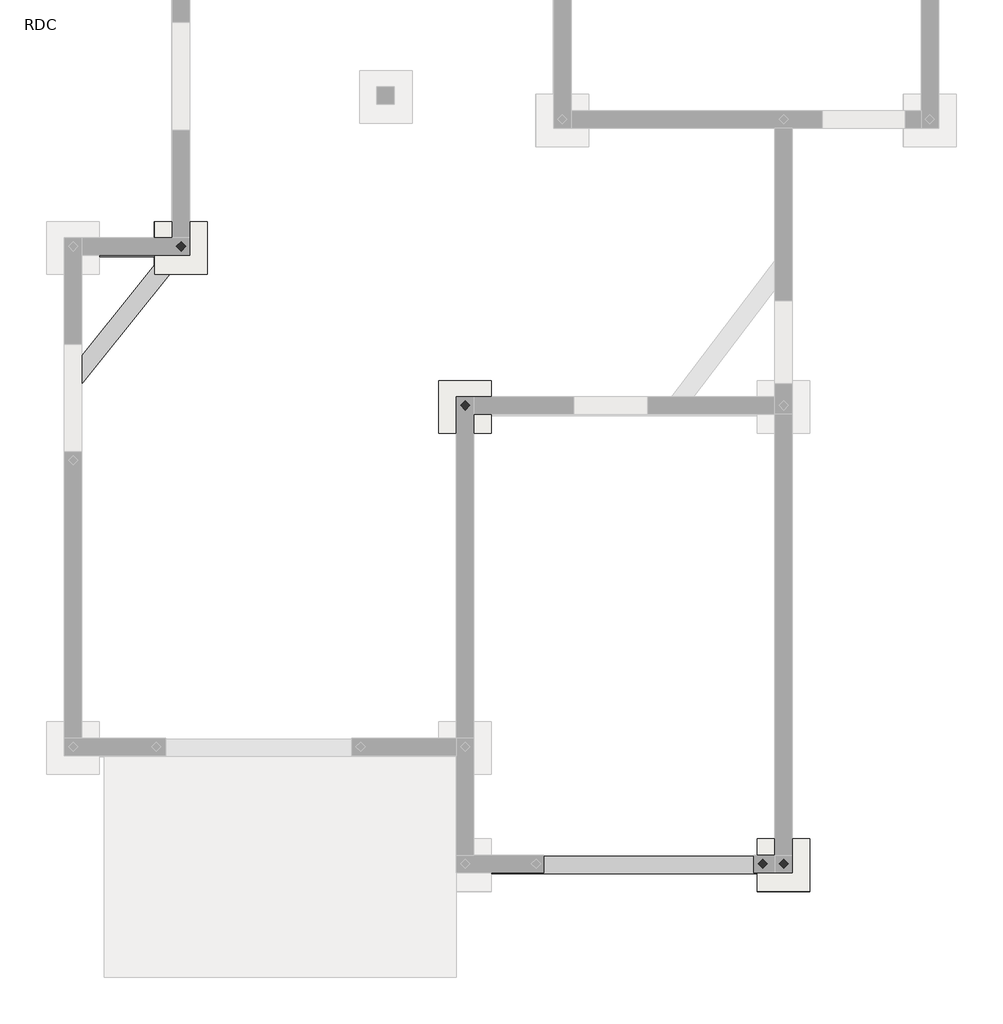
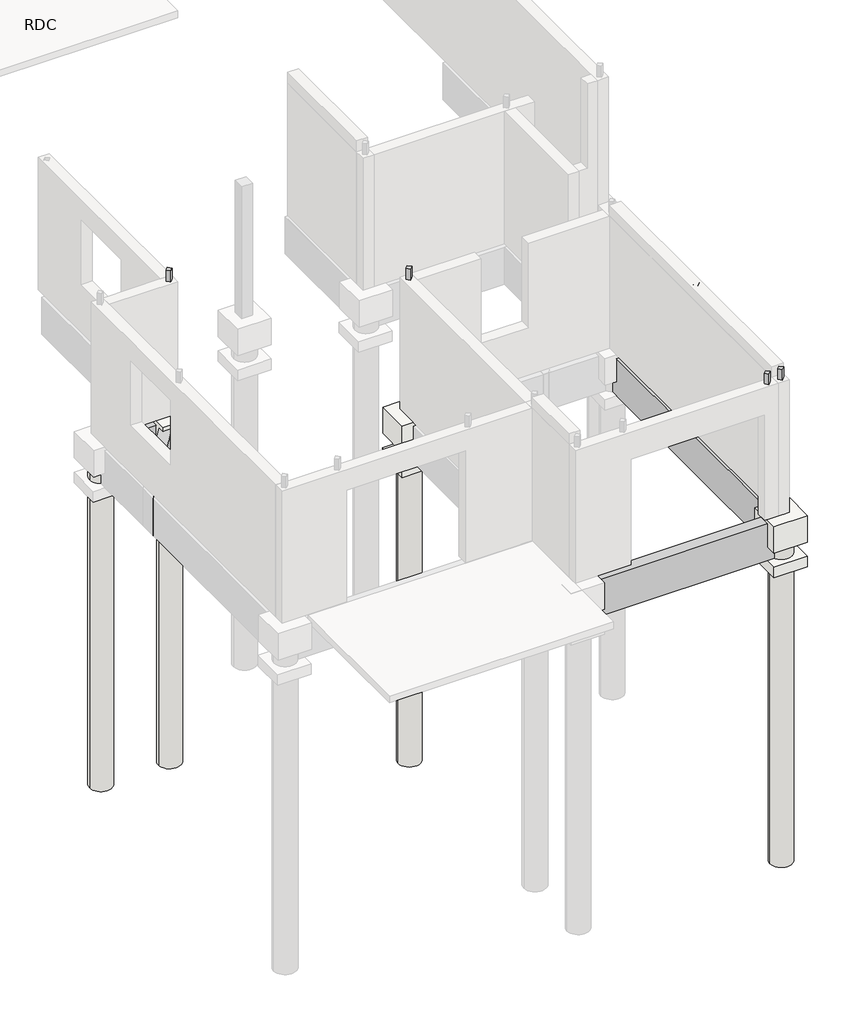
# One storey, part 3 of 5: 10 slabs, 5 columns, 4 beams.
"""IFC4 building model written with IfcOpenShell, lengths in millimetres."""

from ifc_helpers import new_model, si_unit, frame, origin, place, context, project, spatial, polyline, circle_curve, outline, extrude, faceted_brep, element, save
from ifc_brep_helpers import plane_surface, cylinder_surface, revolved_surface, advanced_brep

model = new_model("IFC4")

# Units and contexts
model_context = context("Model", 3, world=origin())
ifc_project = project(units=[si_unit("LENGTHUNIT", "METRE", prefix="MILLI")], contexts=[model_context])

# Site, building, storey
site = spatial("IfcSite", under=ifc_project)
building = spatial("IfcBuilding", under=site)
storey = spatial("IfcBuildingStorey", under=building, Name="RDC", Elevation=0.0)

# Beams
placement = place(None, origin())
element("IfcBeam", 1, ObjectType="Longrine BA : 20x70ht", at=placement, inside=storey, context=model_context, shape_type="AdvancedBrep", body=[
    advanced_brep(
    [(-6246.4904447, -2429.4243416, -767.0), (-6246.4904447, -2429.4243416, -67.0), (-5212.6214092, -1137.6788036, -67.0), (-5212.6214092, -1137.6788036, -500.0), (-5104.1092044, -1002.1005519, -500.0), (-5104.1092044, -1002.1005519, -767.0), (-4957.6914228, -1139.2289701, -767.0), (-6246.4904447, -2749.4913232, -767.0), (-6246.4904447, -2749.4913232, -67.0), (-4957.6914228, -1139.2289701, -500.0), (-5041.8454341, -1244.3733983, -500.0), (-5041.8454341, -1244.3733983, -67.0), (-5212.6214092, -1244.3733983, -67.0), (-5212.6214092, -1244.3733983, -500.0)],
    [
        (0, 1),
        (1, 2),
        (2, 3),
        (3, 4),
        (4, 5),
        (5, 0),
        (5, 6, circle_curve(frame((-4912.6214092, -944.3733983, -767.0), z_axis=(0.0, 0.0, 1.0), x_axis=(1.0, 0.0, 0.0)), 200.0)),
        (6, 7),
        (7, 0),
        (8, 7),
        (6, 9),
        (9, 10),
        (10, 11),
        (11, 8),
        (1, 8),
        (11, 12),
        (12, 2),
        (4, 9, circle_curve(frame((-4912.6214092, -944.3733983, -500.0), z_axis=(0.0, 0.0, 1.0), x_axis=(1.0, 0.0, 0.0)), 200.0)),
        (3, 13),
        (13, 10),
        (12, 13),
    ],
    [
        plane_surface(frame((-6038.5546058, -2169.6233583, -67.0), z_axis=(-0.780729452475571, 0.6248692039436695, 0.0), x_axis=(0.6248692039436695, 0.780729452475571, 0.0))),
        plane_surface(frame((-6038.5546058, -2169.6233583, -767.0), z_axis=(0.0, 0.0, -1.0000000000000002), x_axis=(0.6248692039436695, 0.780729452475571, 0.0))),
        plane_surface(frame((-5882.4087153, -2294.5971991, -767.0), z_axis=(0.780729452475571, -0.6248692039436695, 0.0), x_axis=(0.6248692039436695, 0.780729452475571, 0.0))),
        plane_surface(frame((-5882.4087153, -2294.5971991, -67.0), z_axis=(0.0, 0.0, 1.0000000000000002), x_axis=(0.6248692039436695, 0.780729452475571, 0.0))),
        revolved_surface(polyline([(-4712.6214092, -944.3733983, -500.0), (-4712.6214092, -944.3733983, -767.0)]), (-4912.6214092, -944.3733983, -6600.0), (0.0, 0.0, 1.0)),
        plane_surface(frame((-6246.4904447, -2766.3120846, -67.0), z_axis=(-1.0, 0.0, 0.0), x_axis=(0.0, 1.0, 0.0))),
        plane_surface(frame((-5212.6214092, -644.3733983, -500.0), z_axis=(0.0, 0.0, 1.0), x_axis=(1.0, 0.0, 0.0))),
        plane_surface(frame((-5212.6214092, -644.3733983, 0.0), z_axis=(1.0, 0.0, 0.0), x_axis=(0.0, 0.0, -1.0))),
        plane_surface(frame((-5212.6214092, -1244.3733983, 0.0), z_axis=(0.0, 1.0, 0.0), x_axis=(0.0, 0.0, -1.0))),
    ],
    [
        (0, [[1, 2, 3, 4, 5, 6]]),
        (1, [[7, 8, 9, -6]]),
        (2, [[10, -8, 11, 12, 13, 14]]),
        (3, [[15, -14, 16, 17, -2]]),
        (4, [[-7, -5, 18, -11]]),
        (5, [[-1, -9, -10, -15]]),
        (6, [[19, 20, -12, -18, -4]]),
        (7, [[-19, -3, -17, 21]]),
        (8, [[-20, -21, -16, -13]]),
    ],
),
])
element("IfcBeam", 2, ObjectType="Longrine BA : 20x70ht", at=placement, inside=storey, context=model_context, shape_type="AdvancedBrep", body=[
    advanced_brep(
    [(1796.8177589, -8101.9775185, -767.0), (1796.8177589, -8101.9775185, -500.0), (1670.0228479, -8101.9775185, -500.0), (1670.0228479, -8101.9775185, -67.0), (-1366.4904447, -8101.9775185, -67.0), (-1366.4904447, -8101.9775185, -500.0), (-1493.285364, -8101.9775185, -500.0), (-1493.285364, -8101.9775185, -767.0), (-1466.4904447, -8001.9775185, -767.0), (-1493.285364, -7901.9775185, -767.0), (1796.8177754, -7901.9775185, -767.0), (1770.0228479, -8001.9775328, -767.0), (1796.8177754, -7901.9775185, -500.0), (-1493.285364, -7901.9775185, -500.0), (-1366.4904447, -7901.9775185, -500.0), (-1366.4904447, -7901.9775185, -67.0), (1670.0228479, -7901.9775185, -67.0), (1670.0228479, -7901.9775185, -500.0), (-1466.4904447, -8001.9775185, -500.0), (1770.0228479, -8001.9775328, -500.0)],
    [
        (0, 1),
        (1, 2),
        (2, 3),
        (3, 4),
        (4, 5),
        (5, 6),
        (6, 7),
        (7, 0),
        (7, 8, circle_curve(frame((-1666.4904447, -8001.9775185, -767.0), z_axis=(0.0, 0.0, 1.0), x_axis=(1.0, 0.0, 0.0)), 200.0)),
        (8, 9, circle_curve(frame((-1666.4904447, -8001.9775185, -767.0), z_axis=(0.0, 0.0, 1.0), x_axis=(1.0, 0.0, 0.0)), 200.0)),
        (9, 10),
        (10, 11, circle_curve(frame((1970.0228479, -8001.9775328, -767.0), z_axis=(0.0, 0.0, 1.0), x_axis=(1.0, 0.0, 0.0)), 200.0)),
        (11, 0, circle_curve(frame((1970.0228479, -8001.9775328, -767.0), z_axis=(0.0, 0.0, 1.0), x_axis=(1.0, 0.0, 0.0)), 200.0)),
        (12, 10),
        (9, 13),
        (13, 14),
        (14, 15),
        (15, 16),
        (16, 17),
        (17, 12),
        (3, 16),
        (15, 4),
        (6, 18, circle_curve(frame((-1666.4904447, -8001.9775185, -500.0), z_axis=(0.0, 0.0, 1.0), x_axis=(1.0, 0.0, 0.0)), 200.0)),
        (18, 8),
        (18, 13, circle_curve(frame((-1666.4904447, -8001.9775185, -500.0), z_axis=(0.0, 0.0, 1.0), x_axis=(1.0, 0.0, 0.0)), 200.0)),
        (11, 19),
        (19, 1, circle_curve(frame((1970.0228479, -8001.9775328, -500.0), z_axis=(0.0, 0.0, 1.0), x_axis=(1.0, 0.0, 0.0)), 200.0)),
        (12, 19, circle_curve(frame((1970.0228479, -8001.9775328, -500.0), z_axis=(0.0, 0.0, 1.0), x_axis=(1.0, 0.0, 0.0)), 200.0)),
        (17, 2),
        (5, 14),
    ],
    [
        plane_surface(frame((1961.8663633, -8101.9775185, -417.0), z_axis=(0.0, -1.0, 0.0), x_axis=(0.0, 0.0, -1.0))),
        plane_surface(frame((1961.8663633, -8001.9775185, -767.0), z_axis=(0.0, 0.0, -1.0), x_axis=(0.0, 1.0, 0.0))),
        plane_surface(frame((1961.8663633, -7901.9775185, -417.0), z_axis=(0.0, 1.0, 0.0), x_axis=(0.0, 0.0, 1.0))),
        plane_surface(frame((1961.8663633, -8001.9775185, -67.0), z_axis=(0.0, 0.0, 1.0), x_axis=(0.0, -1.0, 0.0))),
        revolved_surface(polyline([(-1466.4904447, -8001.9775185, -500.0), (-1466.4904447, -8001.9775185, -767.0)]), (-1666.4904447, -8001.9775185, -6600.0), (0.0, 0.0, 1.0)),
        revolved_surface(polyline([(2170.0228478999998, -8001.9775328, -500.0), (2170.0228478999998, -8001.9775328, -767.0)]), (1970.0228479, -8001.9775328, -6600.0), (0.0, 0.0, 1.0)),
        plane_surface(frame((1670.0228479, -7701.9775328, -500.0), z_axis=(0.0, 0.0, 1.0), x_axis=(1.0, 0.0, 0.0))),
        plane_surface(frame((1670.0228479, -7701.9775328, 0.0), z_axis=(1.0, 0.0, 0.0), x_axis=(0.0, 0.0, -1.0))),
        plane_surface(frame((-1966.4904447, -7701.9775185, -500.0), z_axis=(0.0, 0.0, 1.0), x_axis=(1.0, 0.0, 0.0))),
        plane_surface(frame((-1366.4904447, -8301.9775185, 0.0), z_axis=(-1.0, 0.0, 0.0), x_axis=(0.0, 0.0, -1.0))),
    ],
    [
        (0, [[1, 2, 3, 4, 5, 6, 7, 8]]),
        (1, [[9, 10, 11, 12, 13, -8]]),
        (2, [[14, -11, 15, 16, 17, 18, 19, 20]]),
        (3, [[21, -18, 22, -4]]),
        (4, [[-9, -7, 23, 24]]),
        (4, [[-10, -24, 25, -15]]),
        (5, [[-1, -13, 26, 27]]),
        (5, [[-14, 28, -26, -12]]),
        (6, [[29, -2, -27, -28, -20]]),
        (7, [[-29, -19, -21, -3]]),
        (8, [[30, -16, -25, -23, -6]]),
        (9, [[-30, -5, -22, -17]]),
    ],
),
])
element("IfcBeam", 3, ObjectType="Longrine BA : 20x70ht", at=placement, inside=storey, context=model_context, shape_type="AdvancedBrep", body=[
    advanced_brep(
    [(2074.5663639, -2932.4787022, -767.0), (2074.5663639, -2932.4787022, -500.0), (2074.5663639, -3061.9775197, -500.0), (2074.5663639, -3061.9775197, -67.0), (2074.5663639, -7701.9775328, -67.0), (2074.5663639, -7701.9775328, -500.0), (2074.5663639, -7831.4763502, -500.0), (2074.5663639, -7831.4763502, -767.0), (1874.5663639, -7826.2275409, -767.0), (1874.5663639, -2937.7275116, -767.0), (1874.5663639, -2937.7275116, -500.0), (1874.5663639, -7826.2275409, -500.0), (1874.5663639, -7701.9775328, -500.0), (1874.5663639, -7701.9775328, -67.0), (1874.5663639, -3061.9775197, -67.0), (1874.5663639, -3061.9775197, -500.0)],
    [
        (0, 1),
        (1, 2),
        (2, 3),
        (3, 4),
        (4, 5),
        (5, 6),
        (6, 7),
        (7, 0),
        (7, 8, circle_curve(frame((1970.0228479, -8001.9775328, -767.0), z_axis=(0.0, 0.0, 1.0), x_axis=(1.0, 0.0, 0.0)), 200.0)),
        (8, 9),
        (9, 0, circle_curve(frame((1970.0228479, -2761.9775197, -767.0), z_axis=(0.0, 0.0, 1.0), x_axis=(1.0, 0.0, 0.0)), 200.0)),
        (10, 9),
        (8, 11),
        (11, 12),
        (12, 13),
        (13, 14),
        (14, 15),
        (15, 10),
        (3, 14),
        (13, 4),
        (10, 1, circle_curve(frame((1970.0228479, -2761.9775197, -500.0), z_axis=(0.0, 0.0, 1.0), x_axis=(1.0, 0.0, 0.0)), 200.0)),
        (6, 11, circle_curve(frame((1970.0228479, -8001.9775328, -500.0), z_axis=(0.0, 0.0, 1.0), x_axis=(1.0, 0.0, 0.0)), 200.0)),
        (15, 2),
        (5, 12),
    ],
    [
        plane_surface(frame((2074.5663639, -2774.6775203, -417.0), z_axis=(1.0, 0.0, 0.0), x_axis=(0.0, 0.0, -1.0))),
        plane_surface(frame((1974.5663639, -2774.6775203, -767.0), z_axis=(0.0, 0.0, -1.0), x_axis=(-1.0, 0.0, 0.0))),
        plane_surface(frame((1874.5663639, -2774.6775203, -417.0), z_axis=(-1.0, 0.0, 0.0), x_axis=(0.0, 0.0, 1.0))),
        plane_surface(frame((1974.5663639, -2774.6775203, -67.0), z_axis=(0.0, 0.0, 1.0), x_axis=(1.0, 0.0, 0.0))),
        revolved_surface(polyline([(2170.0228478999998, -2761.9775197, -500.0), (2170.0228478999998, -2761.9775197, -767.0)]), (1970.0228479, -2761.9775197, -6600.0), (0.0, 0.0, 1.0)),
        revolved_surface(polyline([(2170.0228478999998, -8001.9775328, -500.0), (2170.0228478999998, -8001.9775328, -767.0)]), (1970.0228479, -8001.9775328, -6600.0), (0.0, 0.0, 1.0)),
        plane_surface(frame((1670.0228479, -2461.9775197, -500.0), z_axis=(0.0, 0.0, 1.0), x_axis=(1.0, 0.0, 0.0))),
        plane_surface(frame((1670.0228479, -3061.9775197, 0.0), z_axis=(0.0, 1.0, 0.0), x_axis=(0.0, 0.0, -1.0))),
        plane_surface(frame((1670.0228479, -7701.9775328, -500.0), z_axis=(0.0, 0.0, 1.0), x_axis=(1.0, 0.0, 0.0))),
        plane_surface(frame((2270.0228479, -7701.9775328, 0.0), z_axis=(0.0, -1.0, 0.0), x_axis=(0.0, 0.0, -1.0))),
    ],
    [
        (0, [[1, 2, 3, 4, 5, 6, 7, 8]]),
        (1, [[9, 10, 11, -8]]),
        (2, [[12, -10, 13, 14, 15, 16, 17, 18]]),
        (3, [[19, -16, 20, -4]]),
        (4, [[-1, -11, -12, 21]]),
        (5, [[-9, -7, 22, -13]]),
        (6, [[23, -2, -21, -18]]),
        (7, [[-23, -17, -19, -3]]),
        (8, [[24, -14, -22, -6]]),
        (9, [[-24, -5, -20, -15]]),
    ],
),
])
element("IfcBeam", 4, ObjectType="Longrine BA : 20x70ht", at=placement, inside=storey, context=model_context, shape_type="AdvancedBrep", body=[
    advanced_brep(
    [(-5085.826475, -1044.3734242, -500.0), (-5212.6214092, -1044.3734242, -500.0), (-5212.6214092, -1044.3734242, -67.0), (-5846.4904447, -1044.3734242, -67.0), (-5846.4904447, -1044.3734242, -500.0), (-5973.2853789, -1044.3734242, -500.0), (-5973.2853789, -1044.3734242, -767.0), (-5085.826475, -1044.3734242, -767.0), (-5112.6214092, -944.3733983, -767.0), (-5946.4904447, -944.3733983, -767.0), (-5973.285349, -844.3734242, -767.0), (-5085.8265049, -844.3734242, -767.0), (-5085.8265049, -844.3734242, -500.0), (-5973.285349, -844.3734242, -500.0), (-5846.4904447, -844.3734242, -500.0), (-5846.4904447, -844.3734242, -67.0), (-5212.6214092, -844.3734242, -67.0), (-5212.6214092, -844.3734242, -500.0), (-5112.6214092, -944.3733983, -500.0), (-5946.4904447, -944.3733983, -500.0)],
    [
        (0, 1),
        (1, 2),
        (2, 3),
        (3, 4),
        (4, 5),
        (5, 6),
        (6, 7),
        (7, 0),
        (8, 7, circle_curve(frame((-4912.6214092, -944.3733983, -767.0), z_axis=(0.0, 0.0, 1.0), x_axis=(1.0, 0.0, 0.0)), 200.0)),
        (6, 9, circle_curve(frame((-6146.4904447, -944.3733983, -767.0), z_axis=(0.0, 0.0, 1.0), x_axis=(1.0, 0.0, 0.0)), 200.0)),
        (9, 10, circle_curve(frame((-6146.4904447, -944.3733983, -767.0), z_axis=(0.0, 0.0, 1.0), x_axis=(1.0, 0.0, 0.0)), 200.0)),
        (10, 11),
        (11, 8, circle_curve(frame((-4912.6214092, -944.3733983, -767.0), z_axis=(0.0, 0.0, 1.0), x_axis=(1.0, 0.0, 0.0)), 200.0)),
        (12, 11),
        (10, 13),
        (13, 14),
        (14, 15),
        (15, 16),
        (16, 17),
        (17, 12),
        (2, 16),
        (15, 3),
        (8, 18),
        (18, 0, circle_curve(frame((-4912.6214092, -944.3733983, -500.0), z_axis=(0.0, 0.0, 1.0), x_axis=(1.0, 0.0, 0.0)), 200.0)),
        (12, 18, circle_curve(frame((-4912.6214092, -944.3733983, -500.0), z_axis=(0.0, 0.0, 1.0), x_axis=(1.0, 0.0, 0.0)), 200.0)),
        (5, 19, circle_curve(frame((-6146.4904447, -944.3733983, -500.0), z_axis=(0.0, 0.0, 1.0), x_axis=(1.0, 0.0, 0.0)), 200.0)),
        (19, 9),
        (19, 13, circle_curve(frame((-6146.4904447, -944.3733983, -500.0), z_axis=(0.0, 0.0, 1.0), x_axis=(1.0, 0.0, 0.0)), 200.0)),
        (17, 1),
        (4, 14),
    ],
    [
        plane_surface(frame((-4942.5210392, -1044.3734242, -417.0), z_axis=(0.0, -1.0, 0.0), x_axis=(0.0, 0.0, -1.0))),
        plane_surface(frame((-4942.5210392, -944.3734242, -767.0), z_axis=(0.0, 0.0, -1.0), x_axis=(0.0, 1.0, 0.0))),
        plane_surface(frame((-4942.5210392, -844.3734242, -417.0), z_axis=(0.0, 1.0, 0.0), x_axis=(0.0, 0.0, 1.0))),
        plane_surface(frame((-4942.5210392, -944.3734242, -67.0), z_axis=(0.0, 0.0, 1.0), x_axis=(0.0, -1.0, 0.0))),
        revolved_surface(polyline([(-4712.6214092, -944.3733983, -500.0), (-4712.6214092, -944.3733983, -767.0)]), (-4912.6214092, -944.3733983, -6600.0), (0.0, 0.0, 1.0)),
        revolved_surface(polyline([(-5946.4904447, -944.3733983, -500.0), (-5946.4904447, -944.3733983, -767.0)]), (-6146.4904447, -944.3733983, -6600.0), (0.0, 0.0, 1.0)),
        plane_surface(frame((-5212.6214092, -644.3733983, -500.0), z_axis=(0.0, 0.0, 1.0), x_axis=(1.0, 0.0, 0.0))),
        plane_surface(frame((-5212.6214092, -644.3733983, 0.0), z_axis=(1.0, 0.0, 0.0), x_axis=(0.0, 0.0, -1.0))),
        plane_surface(frame((-6446.4904447, -644.3733983, -500.0), z_axis=(0.0, 0.0, 1.0), x_axis=(1.0, 0.0, 0.0))),
        plane_surface(frame((-5846.4904447, -1244.3733983, 0.0), z_axis=(-1.0, 0.0, 0.0), x_axis=(0.0, 0.0, -1.0))),
    ],
    [
        (0, [[1, 2, 3, 4, 5, 6, 7, 8]]),
        (1, [[9, -7, 10, 11, 12, 13]]),
        (2, [[14, -12, 15, 16, 17, 18, 19, 20]]),
        (3, [[21, -18, 22, -3]]),
        (4, [[-9, 23, 24, -8]]),
        (4, [[-14, 25, -23, -13]]),
        (5, [[-10, -6, 26, 27]]),
        (5, [[-11, -27, 28, -15]]),
        (6, [[29, -1, -24, -25, -20]]),
        (7, [[-29, -19, -21, -2]]),
        (8, [[30, -16, -28, -26, -5]]),
        (9, [[-30, -4, -22, -17]]),
    ],
),
])

# Columns
element("IfcColumn", 5, ObjectType="CV : CV", at=placement, inside=storey, context=model_context, shape_type="Brep", body=[
    faceted_brep([(-1665.4336406, -2693.1316224, 2710.0), (-1718.4666492, -2746.164631, 2710.0), (-1665.4336406, -2799.1976396, 2710.0), (-1612.400632, -2746.164631, 2710.0), (-1665.4336406, -2693.1316224, 0.0), (-1612.400632, -2746.164631, 0.0), (-1665.4336406, -2799.1976396, 0.0), (-1718.4666492, -2746.164631, 0.0), (-1665.4336406, -2693.1316224, 2500.0), (-1718.4666492, -2746.164631, 2500.0), (-1665.4336406, -2799.1976396, 2500.0), (-1612.400632, -2746.164631, 2500.0)], [[[0, 1, 2, 3]], [[4, 5, 6, 7]], [[1, 0, 8, 4, 7, 9]], [[2, 1, 9, 7, 6, 10]], [[3, 2, 10, 6, 5, 11]], [[0, 3, 11, 5, 4, 8]]]),
    faceted_brep([(-1612.400632, -2746.164631, 2710.0), (-1665.4336406, -2693.1316224, 2710.0), (-1718.4666492, -2746.164631, 2710.0), (-1665.4336406, -2799.1976396, 2710.0), (-1612.400632, -2746.164631, 0.0), (-1665.4336406, -2799.1976396, 0.0), (-1718.4666492, -2746.164631, 0.0), (-1665.4336406, -2693.1316224, 0.0), (-1612.400632, -2746.164631, 2500.0), (-1665.4336406, -2693.1316224, 2500.0), (-1718.4666492, -2746.164631, 2500.0), (-1665.4336406, -2799.1976396, 2500.0)], [[[0, 1, 2, 3]], [[4, 5, 6, 7]], [[1, 0, 8, 4, 7, 9]], [[2, 1, 9, 7, 6, 10]], [[3, 2, 10, 6, 5, 11]], [[0, 3, 11, 5, 4, 8]]]),
])
element("IfcColumn", 6, ObjectType="CV : CV", at=placement, inside=storey, context=model_context, shape_type="Brep", body=[
    faceted_brep([(1974.5663639, -5313.1316158, 2710.0), (1921.5333553, -5366.1646244, 2710.0), (1974.5663639, -5419.197633, 2710.0), (2027.5993725, -5366.1646244, 2710.0), (1974.5663639, -5313.1316158, 0.0), (2027.5993725, -5366.1646244, 0.0), (1974.5663639, -5419.197633, 0.0), (1921.5333553, -5366.1646244, 0.0), (1974.5663639, -5313.1316158, 2510.0), (1921.5333553, -5366.1646244, 2510.0), (1974.5663639, -5419.197633, 2510.0), (2027.5993725, -5366.1646244, 2510.0)], [[[0, 1, 2, 3]], [[4, 5, 6, 7]], [[1, 0, 8, 4, 7, 9]], [[2, 1, 9, 7, 6, 10]], [[3, 2, 10, 6, 5, 11]], [[0, 3, 11, 5, 4, 8]]]),
    faceted_brep([(2027.5993725, -5366.1646244, 2710.0), (1974.5663639, -5313.1316158, 2710.0), (1921.5333553, -5366.1646244, 2710.0), (1974.5663639, -5419.197633, 2710.0), (2027.5993725, -5366.1646244, 0.0), (1974.5663639, -5419.197633, 0.0), (1921.5333553, -5366.1646244, 0.0), (1974.5663639, -5313.1316158, 0.0), (2027.5993725, -5366.1646244, 2510.0), (1974.5663639, -5313.1316158, 2510.0), (1921.5333553, -5366.1646244, 2510.0), (1974.5663639, -5419.197633, 2510.0)], [[[0, 1, 2, 3]], [[4, 5, 6, 7]], [[1, 0, 8, 4, 7, 9]], [[2, 1, 9, 7, 6, 10]], [[3, 2, 10, 6, 5, 11]], [[0, 3, 11, 5, 4, 8]]]),
])
element("IfcColumn", 7, ObjectType="CV : CV", at=placement, inside=storey, context=model_context, shape_type="Brep", body=[
    faceted_brep([(1974.5663639, -7933.1316212, 2710.0), (1921.5333553, -7986.1646298, 2710.0), (1974.5663639, -8039.1976384, 2710.0), (2027.5993725, -7986.1646298, 2710.0), (1974.5663639, -7933.1316212, 0.0), (2027.5993725, -7986.1646298, 0.0), (1974.5663639, -8039.1976384, 0.0), (1921.5333553, -7986.1646298, 0.0), (1974.5663639, -7933.1316212, 2510.0), (1921.5333553, -7986.1646298, 2510.0), (1974.5663639, -8039.1976384, 2510.0), (2027.5993725, -7986.1646298, 2510.0)], [[[0, 1, 2, 3]], [[4, 5, 6, 7]], [[1, 0, 8, 4, 7, 9]], [[2, 1, 9, 7, 6, 10]], [[3, 2, 10, 6, 5, 11]], [[0, 3, 11, 5, 4, 8]]]),
    faceted_brep([(2027.5993725, -7986.1646298, 2710.0), (1974.5663639, -7933.1316212, 2710.0), (1921.5333553, -7986.1646298, 2710.0), (1974.5663639, -8039.1976384, 2710.0), (2027.5993725, -7986.1646298, 0.0), (1974.5663639, -8039.1976384, 0.0), (1921.5333553, -7986.1646298, 0.0), (1974.5663639, -7933.1316212, 0.0), (2027.5993725, -7986.1646298, 2510.0), (1974.5663639, -7933.1316212, 2510.0), (1921.5333553, -7986.1646298, 2510.0), (1974.5663639, -8039.1976384, 2510.0)], [[[0, 1, 2, 3]], [[4, 5, 6, 7]], [[1, 0, 8, 4, 7, 9]], [[2, 1, 9, 7, 6, 10]], [[3, 2, 10, 6, 5, 11]], [[0, 3, 11, 5, 4, 8]]]),
])
element("IfcColumn", 8, ObjectType="CV : CV", at=placement, inside=storey, context=model_context, shape_type="Brep", body=[
    faceted_brep([(1734.5663809, -7933.1316212, 2710.0), (1681.5333723, -7986.1646298, 2710.0), (1734.5663809, -8039.1976384, 2710.0), (1787.5993895, -7986.1646298, 2710.0), (1734.5663809, -7933.1316212, 0.0), (1787.5993895, -7986.1646298, 0.0), (1734.5663809, -8039.1976384, 0.0), (1681.5333723, -7986.1646298, 0.0), (1734.5663809, -7933.1316212, 2510.0), (1681.5333723, -7986.1646298, 2510.0), (1734.5663809, -8039.1976384, 2510.0), (1787.5993895, -7986.1646298, 2510.0)], [[[0, 1, 2, 3]], [[4, 5, 6, 7]], [[1, 0, 8, 4, 7, 9]], [[2, 1, 9, 7, 6, 10]], [[3, 2, 10, 6, 5, 11]], [[0, 3, 11, 5, 4, 8]]]),
    faceted_brep([(1787.5993895, -7986.1646298, 2710.0), (1734.5663809, -7933.1316212, 2710.0), (1681.5333723, -7986.1646298, 2710.0), (1734.5663809, -8039.1976384, 2710.0), (1787.5993895, -7986.1646298, 0.0), (1734.5663809, -8039.1976384, 0.0), (1681.5333723, -7986.1646298, 0.0), (1734.5663809, -7933.1316212, 0.0), (1787.5993895, -7986.1646298, 2510.0), (1734.5663809, -7933.1316212, 2510.0), (1681.5333723, -7986.1646298, 2510.0), (1734.5663809, -8039.1976384, 2510.0)], [[[0, 1, 2, 3]], [[4, 5, 6, 7]], [[1, 0, 8, 4, 7, 9]], [[2, 1, 9, 7, 6, 10]], [[3, 2, 10, 6, 5, 11]], [[0, 3, 11, 5, 4, 8]]]),
])
element("IfcColumn", 9, ObjectType="CV : CV", at=placement, inside=storey, context=model_context, shape_type="Brep", body=[
    faceted_brep([(-4912.6214092, -875.52751, 2710.0), (-4965.6544178, -928.5605185, 2710.0), (-4912.6214092, -981.5935271, 2710.0), (-4859.5884006, -928.5605185, 2710.0), (-4912.6214092, -875.52751, 0.0), (-4859.5884006, -928.5605185, 0.0), (-4912.6214092, -981.5935271, 0.0), (-4965.6544178, -928.5605185, 0.0), (-4912.6214092, -875.52751, 2500.0), (-4965.6544178, -928.5605185, 2500.0), (-4912.6214092, -981.5935271, 2500.0), (-4859.5884006, -928.5605185, 2500.0)], [[[0, 1, 2, 3]], [[4, 5, 6, 7]], [[1, 0, 8, 4, 7, 9]], [[2, 1, 9, 7, 6, 10]], [[3, 2, 10, 6, 5, 11]], [[0, 3, 11, 5, 4, 8]]]),
    faceted_brep([(-4859.5884006, -928.5605185, 2710.0), (-4912.6214092, -875.52751, 2710.0), (-4965.6544178, -928.5605185, 2710.0), (-4912.6214092, -981.5935271, 2710.0), (-4859.5884006, -928.5605185, 0.0), (-4912.6214092, -981.5935271, 0.0), (-4965.6544178, -928.5605185, 0.0), (-4912.6214092, -875.52751, 0.0), (-4859.5884006, -928.5605185, 2500.0), (-4912.6214092, -875.52751, 2500.0), (-4965.6544178, -928.5605185, 2500.0), (-4912.6214092, -981.5935271, 2500.0)], [[[0, 1, 2, 3]], [[4, 5, 6, 7]], [[1, 0, 8, 4, 7, 9]], [[2, 1, 9, 7, 6, 10]], [[3, 2, 10, 6, 5, 11]], [[0, 3, 11, 5, 4, 8]]]),
])

# Slabs
element("IfcSlab", 10, ObjectType="Pieu-Conduite en acier : Diamètre de 400 mm", at=placement, inside=storey, context=model_context, shape_type="AdvancedBrep", body=[
    advanced_brep(
    [(-1866.4904447, -2764.5149728, -6600.0), (-1466.4904447, -2764.5149728, -6600.0), (-1866.4904447, -2764.5149728, -970.0), (-1466.4904447, -2764.5149728, -970.0)],
    [
        (0, 1, circle_curve(frame((-1666.4904447, -2764.5149728, -6600.0), z_axis=(0.0, 0.0, -1.0), x_axis=(1.0, 0.0, 0.0)), 200.0)),
        (1, 0, circle_curve(frame((-1666.4904447, -2764.5149728, -6600.0), z_axis=(0.0, 0.0, -1.0), x_axis=(1.0, 0.0, 0.0)), 200.0)),
        (2, 3, circle_curve(frame((-1666.4904447, -2764.5149728, -970.0), z_axis=(0.0, 0.0, 1.0), x_axis=(1.0, 0.0, 0.0)), 200.0)),
        (3, 2, circle_curve(frame((-1666.4904447, -2764.5149728, -970.0), z_axis=(0.0, 0.0, 1.0), x_axis=(1.0, 0.0, 0.0)), 200.0)),
        (1, 3),
        (2, 0),
    ],
    [
        plane_surface(frame((-1466.4904447, -2764.5149728, -6600.0), z_axis=(0.0, 0.0, -1.0), x_axis=(0.0, -1.0, 0.0))),
        plane_surface(frame((-1969.9771566, -2464.5149728, -970.0), z_axis=(0.0, 0.0, 1.0), x_axis=(1.0, 0.0, 0.0))),
        cylinder_surface(frame((-1666.4904447, -2764.5149728, -6600.0), z_axis=(0.0, 0.0, 1.0), x_axis=(1.0, 0.0, 0.0)), 200.0),
    ],
    [
        (0, [[1, 2]]),
        (1, [[3, 4]]),
        (2, [[-2, 5, -3, 6]]),
        (2, [[-1, -6, -4, -5]]),
    ],
),
    advanced_brep(
    [(-1866.4904447, -2764.5149728, -770.0), (-1466.4904447, -2764.5149728, -770.0), (-1466.4904447, -2764.5149728, -500.0), (-1491.844941, -2861.9775197, -500.0), (-1566.4773454, -2937.71249, -500.0), (-1766.4829046, -2937.7244066, -500.0), (-1866.4904447, -2764.5149728, -500.0), (-1494.7753589, -2661.9775197, -500.0)],
    [
        (0, 1, circle_curve(frame((-1666.4904447, -2764.5149728, -770.0), z_axis=(0.0, 0.0, 1.0), x_axis=(1.0, 0.0, 0.0)), 200.0)),
        (1, 2),
        (2, 3, circle_curve(frame((-1666.4904447, -2764.5149728, -500.0), z_axis=(0.0, 0.0, -1.0), x_axis=(1.0, 0.0, 0.0)), 200.0)),
        (3, 4, circle_curve(frame((-1666.4904447, -2764.5149728, -500.0), z_axis=(0.0, 0.0, -1.0), x_axis=(1.0, 0.0, 0.0)), 200.0)),
        (4, 5, circle_curve(frame((-1666.4904447, -2764.5149728, -500.0), z_axis=(0.0, 0.0, -1.0), x_axis=(1.0, 0.0, 0.0)), 200.0)),
        (5, 6, circle_curve(frame((-1666.4904447, -2764.5149728, -500.0), z_axis=(0.0, 0.0, -1.0), x_axis=(1.0, 0.0, 0.0)), 200.0)),
        (6, 0),
        (1, 0, circle_curve(frame((-1666.4904447, -2764.5149728, -770.0), z_axis=(0.0, 0.0, 1.0), x_axis=(1.0, 0.0, 0.0)), 200.0)),
        (6, 7, circle_curve(frame((-1666.4904447, -2764.5149728, -500.0), z_axis=(0.0, 0.0, -1.0), x_axis=(1.0, 0.0, 0.0)), 200.0)),
        (7, 2, circle_curve(frame((-1666.4904447, -2764.5149728, -500.0), z_axis=(0.0, 0.0, -1.0), x_axis=(1.0, 0.0, 0.0)), 200.0)),
    ],
    [
        cylinder_surface(frame((-1666.4904447, -2764.5149728, -6600.0), z_axis=(0.0, 0.0, 1.0), x_axis=(1.0, 0.0, 0.0)), 200.0),
        plane_surface(frame((-1969.9771566, -2464.5149728, -770.0), z_axis=(0.0, 0.0, -1.0), x_axis=(-1.0, 0.0, 0.0))),
        plane_surface(frame((-1966.4904447, -2464.5149728, -500.0), z_axis=(0.0, 0.0, 1.0), x_axis=(1.0, 0.0, 0.0))),
    ],
    [
        (0, [[1, 2, 3, 4, 5, 6, 7]]),
        (0, [[8, -7, 9, 10, -2]]),
        (1, [[-1, -8]]),
        (2, [[-6, -5, -4, -3, -10, -9]]),
    ],
),
])
element("IfcSlab", 11, ObjectType="Pieu-Conduite en acier : Diamètre de 400 mm", at=placement, inside=storey, context=model_context, shape_type="AdvancedBrep", body=[
    advanced_brep(
    [(-5112.6214092, -944.3733983, -6600.0), (-4712.6214092, -944.3733983, -6600.0), (-5112.6214092, -944.3733983, -970.0), (-4712.6214092, -944.3733983, -970.0)],
    [
        (0, 1, circle_curve(frame((-4912.6214092, -944.3733983, -6600.0), z_axis=(0.0, 0.0, -1.0), x_axis=(1.0, 0.0, 0.0)), 200.0)),
        (1, 0, circle_curve(frame((-4912.6214092, -944.3733983, -6600.0), z_axis=(0.0, 0.0, -1.0), x_axis=(1.0, 0.0, 0.0)), 200.0)),
        (2, 3, circle_curve(frame((-4912.6214092, -944.3733983, -970.0), z_axis=(0.0, 0.0, 1.0), x_axis=(1.0, 0.0, 0.0)), 200.0)),
        (3, 2, circle_curve(frame((-4912.6214092, -944.3733983, -970.0), z_axis=(0.0, 0.0, 1.0), x_axis=(1.0, 0.0, 0.0)), 200.0)),
        (1, 3),
        (2, 0),
    ],
    [
        plane_surface(frame((-4712.6214092, -944.3733983, -6600.0), z_axis=(0.0, 0.0, -1.0), x_axis=(0.0, -1.0, 0.0))),
        plane_surface(frame((-5217.1649573, -644.3733983, -970.0), z_axis=(0.0, 0.0, 1.0), x_axis=(1.0, 0.0, 0.0))),
        cylinder_surface(frame((-4912.6214092, -944.3733983, -6600.0), z_axis=(0.0, 0.0, 1.0), x_axis=(1.0, 0.0, 0.0)), 200.0),
    ],
    [
        (0, [[1, 2]]),
        (1, [[3, 4]]),
        (2, [[-2, 5, -3, 6]]),
        (2, [[-1, -6, -4, -5]]),
    ],
),
    advanced_brep(
    [(-5112.6214092, -944.3733983, -770.0), (-4712.6214092, -944.3733983, -770.0), (-4712.6214092, -944.3733983, -500.0), (-4957.6914228, -1139.2289701, -500.0), (-5085.8333693, -1044.361482, -500.0), (-5104.1092044, -1002.1005519, -500.0), (-5112.6214092, -944.3733983, -500.0), (-5085.8211389, -844.3641306, -500.0), (-5017.1649422, -773.8722262, -500.0), (-4817.1649422, -768.6233971, -500.0)],
    [
        (0, 1, circle_curve(frame((-4912.6214092, -944.3733983, -770.0), z_axis=(0.0, 0.0, 1.0), x_axis=(1.0, 0.0, 0.0)), 200.0)),
        (1, 2),
        (2, 3, circle_curve(frame((-4912.6214092, -944.3733983, -500.0), z_axis=(0.0, 0.0, -1.0), x_axis=(1.0, 0.0, 0.0)), 200.0)),
        (3, 4, circle_curve(frame((-4912.6214092, -944.3733983, -500.0), z_axis=(0.0, 0.0, -1.0), x_axis=(1.0, 0.0, 0.0)), 200.0)),
        (4, 5, circle_curve(frame((-4912.6214092, -944.3733983, -500.0), z_axis=(0.0, 0.0, -1.0), x_axis=(1.0, 0.0, 0.0)), 200.0)),
        (5, 6, circle_curve(frame((-4912.6214092, -944.3733983, -500.0), z_axis=(0.0, 0.0, -1.0), x_axis=(1.0, 0.0, 0.0)), 200.0)),
        (6, 0),
        (1, 0, circle_curve(frame((-4912.6214092, -944.3733983, -770.0), z_axis=(0.0, 0.0, 1.0), x_axis=(1.0, 0.0, 0.0)), 200.0)),
        (6, 7, circle_curve(frame((-4912.6214092, -944.3733983, -500.0), z_axis=(0.0, 0.0, -1.0), x_axis=(1.0, 0.0, 0.0)), 200.0)),
        (7, 8, circle_curve(frame((-4912.6214092, -944.3733983, -500.0), z_axis=(0.0, 0.0, -1.0), x_axis=(1.0, 0.0, 0.0)), 200.0)),
        (8, 9, circle_curve(frame((-4912.6214092, -944.3733983, -500.0), z_axis=(0.0, 0.0, -1.0), x_axis=(1.0, 0.0, 0.0)), 200.0)),
        (9, 2, circle_curve(frame((-4912.6214092, -944.3733983, -500.0), z_axis=(0.0, 0.0, -1.0), x_axis=(1.0, 0.0, 0.0)), 200.0)),
    ],
    [
        cylinder_surface(frame((-4912.6214092, -944.3733983, -6600.0), z_axis=(0.0, 0.0, 1.0), x_axis=(1.0, 0.0, 0.0)), 200.0),
        plane_surface(frame((-5217.1649573, -644.3733983, -770.0), z_axis=(0.0, 0.0, -1.0), x_axis=(-1.0, 0.0, 0.0))),
        plane_surface(frame((-5212.6214092, -644.3733983, -500.0), z_axis=(0.0, 0.0, 1.0), x_axis=(1.0, 0.0, 0.0))),
    ],
    [
        (0, [[1, 2, 3, 4, 5, 6, 7]]),
        (0, [[8, -7, 9, 10, 11, 12, -2]]),
        (1, [[-1, -8]]),
        (2, [[-6, -5, -4, -3, -12, -11, -10, -9]]),
    ],
),
])
element("IfcSlab", 12, ObjectType="Pieu-Conduite en acier : Diamètre de 400 mm", at=placement, inside=storey, context=model_context, shape_type="AdvancedBrep", body=[
    advanced_brep(
    [(-6346.4904447, -944.3733983, -6600.0), (-5946.4904447, -944.3733983, -6600.0), (-6346.4904447, -944.3733983, -970.0), (-5946.4904447, -944.3733983, -970.0)],
    [
        (0, 1, circle_curve(frame((-6146.4904447, -944.3733983, -6600.0), z_axis=(0.0, 0.0, -1.0), x_axis=(1.0, 0.0, 0.0)), 200.0)),
        (1, 0, circle_curve(frame((-6146.4904447, -944.3733983, -6600.0), z_axis=(0.0, 0.0, -1.0), x_axis=(1.0, 0.0, 0.0)), 200.0)),
        (2, 3, circle_curve(frame((-6146.4904447, -944.3733983, -970.0), z_axis=(0.0, 0.0, 1.0), x_axis=(1.0, 0.0, 0.0)), 200.0)),
        (3, 2, circle_curve(frame((-6146.4904447, -944.3733983, -970.0), z_axis=(0.0, 0.0, 1.0), x_axis=(1.0, 0.0, 0.0)), 200.0)),
        (1, 3),
        (2, 0),
    ],
    [
        plane_surface(frame((-5946.4904447, -944.3733983, -6600.0), z_axis=(0.0, 0.0, -1.0), x_axis=(0.0, -1.0, 0.0))),
        plane_surface(frame((-6451.0339778, -644.3734242, -970.0), z_axis=(0.0, 0.0, 1.0), x_axis=(1.0, 0.0, 0.0))),
        cylinder_surface(frame((-6146.4904447, -944.3733983, -6600.0), z_axis=(0.0, 0.0, 1.0), x_axis=(1.0, 0.0, 0.0)), 200.0),
    ],
    [
        (0, [[1, 2]]),
        (1, [[3, 4]]),
        (2, [[-2, 5, -3, 6]]),
        (2, [[-1, -6, -4, -5]]),
    ],
),
    advanced_brep(
    [(-6346.4904447, -944.3733983, -770.0), (-5946.4904447, -944.3733983, -770.0), (-5946.4904447, -944.3733983, -500.0), (-5973.2937962, -1044.3880018, -500.0), (-6046.4904447, -1117.578479, -500.0), (-6246.4904447, -1117.578479, -500.0), (-6346.4904447, -944.3733983, -500.0), (-5973.285349, -844.3734242, -500.0)],
    [
        (0, 1, circle_curve(frame((-6146.4904447, -944.3733983, -770.0), z_axis=(0.0, 0.0, 1.0), x_axis=(1.0, 0.0, 0.0)), 200.0)),
        (1, 2),
        (2, 3, circle_curve(frame((-6146.4904447, -944.3733983, -500.0), z_axis=(0.0, 0.0, -1.0), x_axis=(1.0, 0.0, 0.0)), 200.0)),
        (3, 4, circle_curve(frame((-6146.4904447, -944.3733983, -500.0), z_axis=(0.0, 0.0, -1.0), x_axis=(1.0, 0.0, 0.0)), 200.0)),
        (4, 5, circle_curve(frame((-6146.4904447, -944.3733983, -500.0), z_axis=(0.0, 0.0, -1.0), x_axis=(1.0, 0.0, 0.0)), 200.0)),
        (5, 6, circle_curve(frame((-6146.4904447, -944.3733983, -500.0), z_axis=(0.0, 0.0, -1.0), x_axis=(1.0, 0.0, 0.0)), 200.0)),
        (6, 0),
        (1, 0, circle_curve(frame((-6146.4904447, -944.3733983, -770.0), z_axis=(0.0, 0.0, 1.0), x_axis=(1.0, 0.0, 0.0)), 200.0)),
        (6, 7, circle_curve(frame((-6146.4904447, -944.3733983, -500.0), z_axis=(0.0, 0.0, -1.0), x_axis=(1.0, 0.0, 0.0)), 200.0)),
        (7, 2, circle_curve(frame((-6146.4904447, -944.3733983, -500.0), z_axis=(0.0, 0.0, -1.0), x_axis=(1.0, 0.0, 0.0)), 200.0)),
    ],
    [
        cylinder_surface(frame((-6146.4904447, -944.3733983, -6600.0), z_axis=(0.0, 0.0, 1.0), x_axis=(1.0, 0.0, 0.0)), 200.0),
        plane_surface(frame((-6451.0339778, -644.3734242, -770.0), z_axis=(0.0, 0.0, -1.0), x_axis=(-1.0, 0.0, 0.0))),
        plane_surface(frame((-6446.4904447, -644.3733983, -500.0), z_axis=(0.0, 0.0, 1.0), x_axis=(1.0, 0.0, 0.0))),
    ],
    [
        (0, [[1, 2, 3, 4, 5, 6, 7]]),
        (0, [[8, -7, 9, 10, -2]]),
        (1, [[-1, -8]]),
        (2, [[-6, -5, -4, -3, -10, -9]]),
    ],
),
])
element("IfcSlab", 13, ObjectType="Pieu-Conduite en acier : Diamètre de 400 mm", at=placement, inside=storey, context=model_context, shape_type="AdvancedBrep", body=[
    advanced_brep(
    [(1770.0228479, -8001.9775328, -6600.0), (2170.0228479, -8001.9775328, -6600.0), (1770.0228479, -8001.9775328, -970.0), (2170.0228479, -8001.9775328, -970.0)],
    [
        (0, 1, circle_curve(frame((1970.0228479, -8001.9775328, -6600.0), z_axis=(0.0, 0.0, -1.0), x_axis=(1.0, 0.0, 0.0)), 200.0)),
        (1, 0, circle_curve(frame((1970.0228479, -8001.9775328, -6600.0), z_axis=(0.0, 0.0, -1.0), x_axis=(1.0, 0.0, 0.0)), 200.0)),
        (2, 3, circle_curve(frame((1970.0228479, -8001.9775328, -970.0), z_axis=(0.0, 0.0, 1.0), x_axis=(1.0, 0.0, 0.0)), 200.0)),
        (3, 2, circle_curve(frame((1970.0228479, -8001.9775328, -970.0), z_axis=(0.0, 0.0, 1.0), x_axis=(1.0, 0.0, 0.0)), 200.0)),
        (1, 3),
        (2, 0),
    ],
    [
        plane_surface(frame((2170.0228479, -8001.9775328, -6600.0), z_axis=(0.0, 0.0, -1.0), x_axis=(0.0, -1.0, 0.0))),
        plane_surface(frame((1670.0228479, -7701.9775328, -970.0), z_axis=(0.0, 0.0, 1.0), x_axis=(1.0, 0.0, 0.0))),
        cylinder_surface(frame((1970.0228479, -8001.9775328, -6600.0), z_axis=(0.0, 0.0, 1.0), x_axis=(1.0, 0.0, 0.0)), 200.0),
    ],
    [
        (0, [[1, 2]]),
        (1, [[3, 4]]),
        (2, [[-2, 5, -3, 6]]),
        (2, [[-1, -6, -4, -5]]),
    ],
),
    advanced_brep(
    [(1770.0228479, -8001.9775328, -770.0), (2170.0228479, -8001.9775328, -770.0), (2170.0228479, -8001.9775328, -500.0), (1796.8177589, -8101.9775185, -500.0), (1770.0228479, -8001.9775328, -500.0), (1796.8177754, -7901.9775185, -500.0), (1874.5489366, -7826.2370074, -500.0), (2074.5557716, -7831.469856, -500.0)],
    [
        (0, 1, circle_curve(frame((1970.0228479, -8001.9775328, -770.0), z_axis=(0.0, 0.0, 1.0), x_axis=(1.0, 0.0, 0.0)), 200.0)),
        (1, 2),
        (2, 3, circle_curve(frame((1970.0228479, -8001.9775328, -500.0), z_axis=(0.0, 0.0, -1.0), x_axis=(1.0, 0.0, 0.0)), 200.0)),
        (3, 4, circle_curve(frame((1970.0228479, -8001.9775328, -500.0), z_axis=(0.0, 0.0, -1.0), x_axis=(1.0, 0.0, 0.0)), 200.0)),
        (4, 0),
        (1, 0, circle_curve(frame((1970.0228479, -8001.9775328, -770.0), z_axis=(0.0, 0.0, 1.0), x_axis=(1.0, 0.0, 0.0)), 200.0)),
        (4, 5, circle_curve(frame((1970.0228479, -8001.9775328, -500.0), z_axis=(0.0, 0.0, -1.0), x_axis=(1.0, 0.0, 0.0)), 200.0)),
        (5, 6, circle_curve(frame((1970.0228479, -8001.9775328, -500.0), z_axis=(0.0, 0.0, -1.0), x_axis=(1.0, 0.0, 0.0)), 200.0)),
        (6, 7, circle_curve(frame((1970.0228479, -8001.9775328, -500.0), z_axis=(0.0, 0.0, -1.0), x_axis=(1.0, 0.0, 0.0)), 200.0)),
        (7, 2, circle_curve(frame((1970.0228479, -8001.9775328, -500.0), z_axis=(0.0, 0.0, -1.0), x_axis=(1.0, 0.0, 0.0)), 200.0)),
    ],
    [
        cylinder_surface(frame((1970.0228479, -8001.9775328, -6600.0), z_axis=(0.0, 0.0, 1.0), x_axis=(1.0, 0.0, 0.0)), 200.0),
        plane_surface(frame((1670.0228479, -7701.9775328, -770.0), z_axis=(0.0, 0.0, -1.0), x_axis=(-1.0, 0.0, 0.0))),
        plane_surface(frame((1670.0228479, -7701.9775328, -500.0), z_axis=(0.0, 0.0, 1.0), x_axis=(1.0, 0.0, 0.0))),
    ],
    [
        (0, [[1, 2, 3, 4, 5]]),
        (0, [[6, -5, 7, 8, 9, 10, -2]]),
        (1, [[-1, -6]]),
        (2, [[-4, -3, -10, -9, -8, -7]]),
    ],
),
])
element("IfcSlab", 14, ObjectType="Tête de pieux-1 poteau : 60x60x50", at=placement, inside=storey, context=model_context, shape_type="Brep", body=[
    faceted_brep([(-1366.4904447, -2464.5149728, 0.0), (-1966.4904447, -2464.5149728, 0.0), (-1966.4904447, -3064.5149728, 0.0), (-1366.4904447, -3064.5149728, 0.0), (-1366.4904447, -2464.5149728, -500.0), (-1366.4904447, -2661.9775197, -500.0), (-1366.4904447, -2861.9775197, -500.0), (-1366.4904447, -3064.5149728, -500.0), (-1566.4904447, -3064.5149728, -500.0), (-1766.4904447, -3064.5149728, -500.0), (-1966.4904447, -3064.5149728, -500.0), (-1966.4904447, -2464.5149728, -500.0)], [[[0, 1, 2, 3]], [[4, 5, 6, 7, 8, 9, 10, 11]], [[1, 0, 4, 11]], [[2, 1, 11, 10]], [[3, 2, 10, 9, 8, 7]], [[0, 3, 7, 6, 5, 4]]]),
])
element("IfcSlab", 15, ObjectType="Tête de pieux-1 poteau : 60x60x50", at=placement, inside=storey, context=model_context, shape_type="Brep", body=[
    faceted_brep([(-4612.6214092, -644.3733983, 0.0), (-5212.6214092, -644.3733983, 0.0), (-5212.6214092, -1244.3733983, 0.0), (-4612.6214092, -1244.3733983, 0.0), (-4612.6214092, -644.3733983, -500.0), (-4612.6214092, -1244.3733983, -500.0), (-5041.8454341, -1244.3733983, -500.0), (-5212.6214092, -1244.3733983, -500.0), (-5212.6214092, -1137.6788036, -500.0), (-5212.6214092, -1044.3734242, -500.0), (-5212.6214092, -844.3734242, -500.0), (-5212.6214092, -644.3733983, -500.0), (-5017.1649422, -644.3733983, -500.0), (-4817.1649422, -644.3733983, -500.0), (-5212.6214092, -1244.3733983, -67.0)], [[[0, 1, 2, 3]], [[4, 5, 6, 7, 8, 9, 10, 11, 12, 13]], [[1, 0, 4, 13, 12, 11]], [[2, 1, 11, 10, 9, 8, 7, 14]], [[3, 2, 14, 7, 6, 5]], [[0, 3, 5, 4]]]),
])
element("IfcSlab", 16, ObjectType="Tête de pieux-1 poteau : 60x60x50", at=placement, inside=storey, context=model_context, shape_type="Brep", body=[
    faceted_brep([(2270.0228479, -7701.9775328, 0.0), (1670.0228479, -7701.9775328, 0.0), (1670.0228479, -8301.9775328, 0.0), (2270.0228479, -8301.9775328, 0.0), (2270.0228479, -7701.9775328, -500.0), (2270.0228479, -8301.9775328, -500.0), (1670.0228479, -8301.9775328, -500.0), (1670.0228479, -8101.9775185, -500.0), (1670.0228479, -7901.9775185, -500.0), (1670.0228479, -7701.9775328, -500.0), (1874.5663639, -7701.9775328, -500.0), (2074.5663639, -7701.9775328, -500.0)], [[[0, 1, 2, 3]], [[4, 5, 6, 7, 8, 9, 10, 11]], [[1, 0, 4, 11, 10, 9]], [[2, 1, 9, 8, 7, 6]], [[3, 2, 6, 5]], [[0, 3, 5, 4]]]),
])
element("IfcSlab", 17, ObjectType="M_Base-Rectangulaire : 60x60x20", at=placement, inside=storey, context=model_context, shape_type="SweptSolid", body=[
    extrude(outline(polyline([(-1369.9771566, -2464.5149728), (-1369.9771566, -3064.5149728), (-1969.9771566, -3064.5149728), (-1969.9771566, -2464.5149728), (-1369.9771566, -2464.5149728)])), frame((0.0, 0.0, -970.0), z_axis=(0.0, 0.0, 1.0), x_axis=(1.0, 0.0, 0.0)), (0.0, 0.0, 1.0), 200.0),
    extrude(outline(polyline([(-1369.9771566, -2464.5149728), (-1369.9771566, -3064.5149728), (-1969.9771566, -3064.5149728), (-1969.9771566, -2464.5149728), (-1369.9771566, -2464.5149728)])), frame((0.0, 0.0, -970.0), z_axis=(0.0, 0.0, 1.0), x_axis=(1.0, 0.0, 0.0)), (0.0, 0.0, 1.0), 200.0),
])
element("IfcSlab", 18, ObjectType="M_Base-Rectangulaire : 60x60x20", at=placement, inside=storey, context=model_context, shape_type="SweptSolid", body=[
    extrude(outline(polyline([(2270.0228479, -7701.9775328), (2270.0228479, -8301.9775328), (1670.0228479, -8301.9775328), (1670.0228479, -7701.9775328), (2270.0228479, -7701.9775328)])), frame((0.0, 0.0, -970.0), z_axis=(0.0, 0.0, 1.0), x_axis=(1.0, 0.0, 0.0)), (0.0, 0.0, 1.0), 200.0),
    extrude(outline(polyline([(2270.0228479, -7701.9775328), (2270.0228479, -8301.9775328), (1670.0228479, -8301.9775328), (1670.0228479, -7701.9775328), (2270.0228479, -7701.9775328)])), frame((0.0, 0.0, -970.0), z_axis=(0.0, 0.0, 1.0), x_axis=(1.0, 0.0, 0.0)), (0.0, 0.0, 1.0), 200.0),
])
element("IfcSlab", 19, ObjectType="M_Base-Rectangulaire : 60x60x20", at=placement, inside=storey, context=model_context, shape_type="SweptSolid", body=[
    extrude(outline(polyline([(-4617.1649573, -644.3733983), (-4617.1649573, -1244.3733983), (-5217.1649573, -1244.3733983), (-5217.1649573, -644.3733983), (-4617.1649573, -644.3733983)])), frame((0.0, 0.0, -970.0), z_axis=(0.0, 0.0, 1.0), x_axis=(1.0, 0.0, 0.0)), (0.0, 0.0, 1.0), 200.0),
    extrude(outline(polyline([(-4617.1649573, -644.3733983), (-4617.1649573, -1244.3733983), (-5217.1649573, -1244.3733983), (-5217.1649573, -644.3733983), (-4617.1649573, -644.3733983)])), frame((0.0, 0.0, -970.0), z_axis=(0.0, 0.0, 1.0), x_axis=(1.0, 0.0, 0.0)), (0.0, 0.0, 1.0), 200.0),
])

save(model, "model.ifc")

# Revit data of these elements
# Type "Longrine BA : 20x70ht"
#   Length [instance default] = 1.524 m
#   b = 0.200 m
#   h = 0.700 m
#   Structural Material = Maçonnerie - Béton
#   Assembly Code = ""
# Type "CV : CV"
#   Structural Material [instance default] = Béton coulé sur place
#   Default Elevation = 0
# Type "Pieu-Conduite en acier : Diamètre de 400 mm"
#   Assembly Code = "A1020130"
#   Rayon = 0.200 m
#   Enrobage minimum = 0.150 m
#   Diameter = 0.400 m
#   Depth = 6.000 m
#   Structural Material [instance default] = Métal - Acier - 345 MPa
# Type "Tête de pieux-1 poteau : 60x60x50"
#   Assembly Code = "A1010130"
#   Width = 0.600 m
#   Length = 0.600 m
#   Foundation Thickness = 0.500 m
#   Coupure = 0.050 m
#   Structural Material [instance default] = Béton - Béton coulé sur place
#   Type de pieu = Pieu-Conduite en acier : Diamètre de 400 mm
# Type "M_Base-Rectangulaire : 60x60x20"
#   Length = 0.600 m
#   Width = 0.600 m
#   Foundation Thickness = 0.200 m
#   Structural Material [instance default] = Béton - Béton coulé sur place
#   Assembly Code = ""
# Elements 1, 2, 3, 4 (IfcBeam, "Longrine BA : 20x70ht")
#   Phase Created = Nouvelle construction
#   Materials on its faces: "Maçonnerie - Béton"
# Elements 5, 6, 7, 8, 9 (IfcColumn, "CV : CV")
#   Structural Material = Béton coulé sur place
#   Phase Created = Nouvelle construction
#   Materials on its faces: "Béton coulé sur place"
# Elements 10, 11, 12, 13 (IfcSlab, "Pieu-Conduite en acier : Diamètre de 400 mm")
#   Structural Material = none
#   Phase Created = Nouvelle construction
# Elements 14, 15, 16 (IfcSlab, "Tête de pieux-1 poteau : 60x60x50")
#   Structural Material = Béton - Béton coulé sur place
#   Phase Created = Nouvelle construction
#   Materials on its faces: "Béton - Béton coulé sur place"
# Elements 17, 18, 19 (IfcSlab, "M_Base-Rectangulaire : 60x60x20")
#   Structural Material = Béton - Béton coulé sur place
#   Phase Created = Nouvelle construction
#   Materials on its faces: "Béton - Béton coulé sur place"
# Materials
#   "Maçonnerie - Béton": class "Béton", colour RGB 153 162 160, transparency 0, Cost = 0
#   "Béton coulé sur place": class "Béton", colour RGB 0 0 0, transparency 0, Description = "Matériau physique.", Cost = 0
#   "Métal - Acier - 345 MPa": class "Métal", colour RGB 247 247 247, transparency 0, Cost = 0
#   "Béton - Béton coulé sur place": class "Béton", colour RGB 192 192 192, transparency 0, Cost = 0
